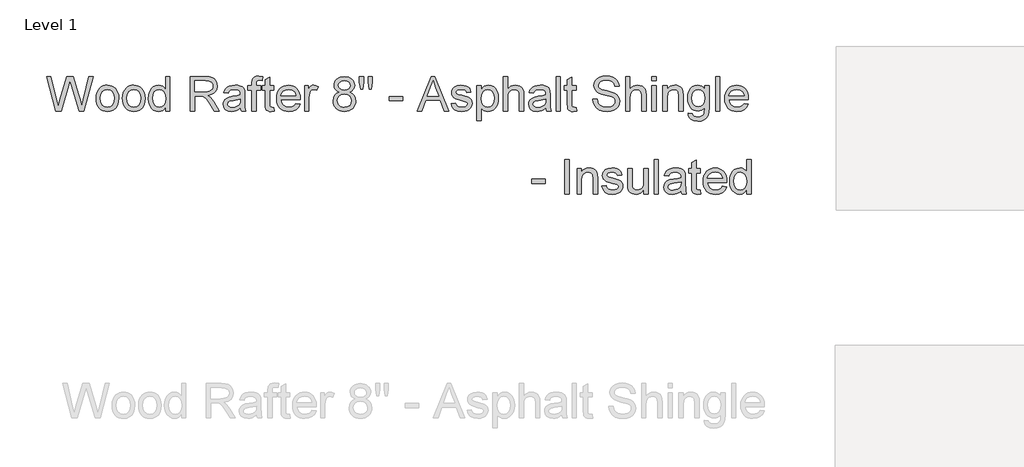
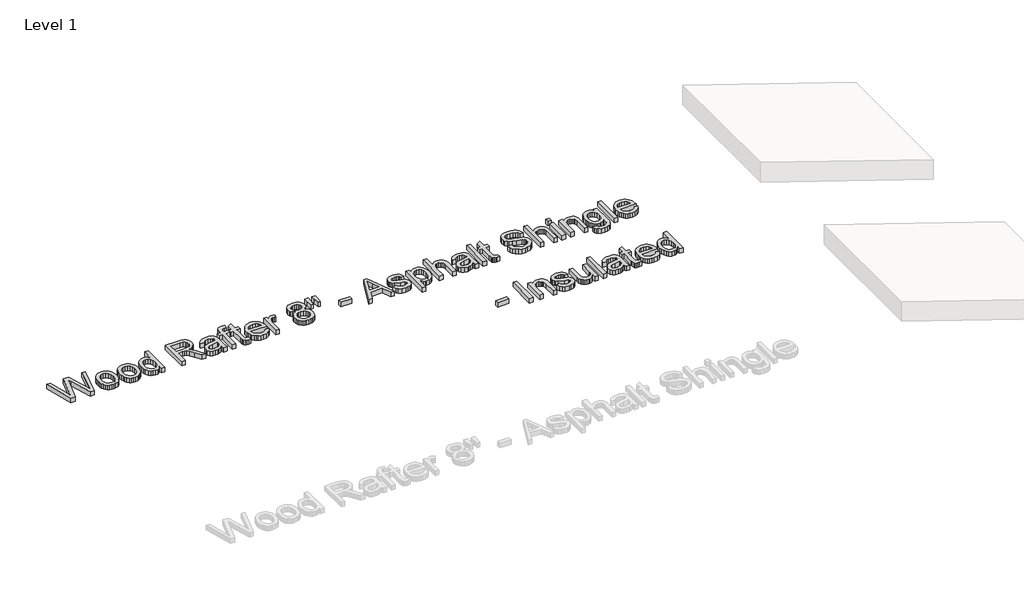
# One storey, part 9 of 42: 1 proxy.
"""IFC4 building model written with IfcOpenShell, lengths in millimetres."""

from ifc_helpers import new_model, si_unit, origin, origin_with_axes, place, context, project, spatial, polyline, outline, extrude, element, save

model = new_model("IFC4")

# Units and contexts
model_context = context("Model", 3, world=origin())
ifc_project = project(units=[si_unit("LENGTHUNIT", "METRE", prefix="MILLI")], contexts=[model_context])

# Site, building, storey
site = spatial("IfcSite", under=ifc_project)
building = spatial("IfcBuilding", under=site)
storey = spatial("IfcBuildingStorey", under=building, Name="Level 1", Elevation=0.0)

# Proxy
placement = place(None, origin())
element("IfcBuildingElementProxy", 1, Name="8\" Arial", ObjectType="8\" Arial", at=placement, inside=storey, context=model_context, shape_type="SweptSolid", body=[
    extrude(outline(polyline([(-8268.0994706, -5719.6737469), (-8351.1564638, -5415.1066528), (-8311.8958618, -5415.1066528), (-8263.7123957, -5615.2762371), (-8248.8409556, -5677.0670709), (-8232.9285147, -5622.4145284), (-8172.5504677, -5415.1066528), (-8115.964638, -5415.1066528), (-8072.0938895, -5565.3825554), (-8053.3001071, -5621.150456), (-8039.4510784, -5677.0670709), (-8025.0257815, -5617.0608099), (-7976.3961722, -5415.1066528), (-7937.1355703, -5415.1066528), (-8020.2669207, -5719.6737469), (-8060.9403094, -5719.6737469), (-8133.9590805, -5484.7049927), (-8144.146017, -5451.9134672), (-8155.5970259, -5491.3971407), (-8222.1467206, -5719.6737469), (-8268.0994706, -5719.6737469)])), origin_with_axes(), (0.0, 0.0, 1.0), 50.8),
    extrude(outline(polyline([(-7913.341266, -5607.840517), (-7911.2825011, -5578.87374), (-7905.1062061, -5553.9129572), (-7894.8123811, -5532.9581686), (-7880.4010261, -5516.0093742), (-7865.8920774, -5505.1764595), (-7849.8773953, -5497.4386633), (-7832.3569798, -5492.7959856), (-7813.3308311, -5491.2484263), (-7792.3272456, -5493.1329167), (-7773.3359518, -5498.7863876), (-7756.3569497, -5508.2088391), (-7741.3902394, -5521.4002712), (-7729.1747456, -5537.9145408), (-7720.4493928, -5557.3055045), (-7715.2141811, -5579.5731625), (-7713.4691106, -5604.7175146), (-7716.5549344, -5643.1787767), (-7725.8124059, -5672.4569245), (-7740.9719802, -5694.383004), (-7761.7641124, -5710.7880614), (-7786.4599977, -5721.0214712), (-7813.3308311, -5724.4326077), (-7834.6411401, -5722.5550884), (-7853.8090322, -5716.9225305), (-7870.8345075, -5707.5349339), (-7885.717566, -5694.3922987), (-7897.8029348, -5677.7176964), (-7906.435341, -5657.7341987), (-7911.6147848, -5634.4418056), (-7913.341266, -5607.840517)]), holes=[polyline([(-7875.2703793, -5607.7661598), (-7870.8647151, -5642.2214277), (-7857.6477227, -5666.7685986), (-7837.7571715, -5681.4634404), (-7813.3308311, -5686.361721), (-7789.0160265, -5681.4355564), (-7769.1626539, -5666.6570628), (-7755.9456615, -5641.7845792), (-7751.5399973, -5606.5764446), (-7755.9735454, -5573.124999), (-7769.2741897, -5548.9124355), (-7789.1554462, -5534.2175937), (-7813.3308311, -5529.3193131), (-7837.7571715, -5534.1990044), (-7857.6477227, -5548.8380783), (-7870.8647151, -5573.3294813), (-7875.2703793, -5607.7661598)])]), origin_with_axes(), (0.0, 0.0, 1.0), 50.8),
    extrude(outline(polyline([(-7680.1570847, -5607.840517), (-7678.0983197, -5578.87374), (-7671.9220247, -5553.9129572), (-7661.6281997, -5532.9581686), (-7647.2168447, -5516.0093742), (-7632.707896, -5505.1764595), (-7616.6932139, -5497.4386633), (-7599.1727984, -5492.7959856), (-7580.1466497, -5491.2484263), (-7559.1430642, -5493.1329167), (-7540.1517704, -5498.7863876), (-7523.1727683, -5508.2088391), (-7508.206058, -5521.4002712), (-7495.9905642, -5537.9145408), (-7487.2652114, -5557.3055045), (-7482.0299997, -5579.5731625), (-7480.2849292, -5604.7175146), (-7483.370753, -5643.1787767), (-7492.6282245, -5672.4569245), (-7507.7877988, -5694.383004), (-7528.579931, -5710.7880614), (-7553.2758163, -5721.0214712), (-7580.1466497, -5724.4326077), (-7601.4569587, -5722.5550884), (-7620.6248508, -5716.9225305), (-7637.6503261, -5707.5349339), (-7652.5333846, -5694.3922987), (-7664.6187534, -5677.7176964), (-7673.2511596, -5657.7341987), (-7678.4306034, -5634.4418056), (-7680.1570847, -5607.840517)]), holes=[polyline([(-7642.0861979, -5607.7661598), (-7637.6805338, -5642.2214277), (-7624.4635413, -5666.7685986), (-7604.5729901, -5681.4634404), (-7580.1466497, -5686.361721), (-7555.8318451, -5681.4355564), (-7535.9784725, -5666.6570628), (-7522.7614801, -5641.7845792), (-7518.3558159, -5606.5764446), (-7522.789364, -5573.124999), (-7536.0900083, -5548.9124355), (-7555.9712648, -5534.2175937), (-7580.1466497, -5529.3193131), (-7604.5729901, -5534.1990044), (-7624.4635413, -5548.8380783), (-7637.6805338, -5573.3294813), (-7642.0861979, -5607.7661598)])]), origin_with_axes(), (0.0, 0.0, 1.0), 50.8),
    extrude(outline(polyline([(-7299.4482171, -5719.6737469), (-7299.4482171, -5683.759219), (-7310.8388107, -5701.5538266), (-7324.6367188, -5714.2642605), (-7340.8419412, -5721.8905209), (-7359.454478, -5724.4326077), (-7384.0667115, -5720.7519263), (-7406.5969433, -5709.709882), (-7425.6695653, -5692.0779308), (-7439.9089692, -5668.6275286), (-7448.7760654, -5640.3067298), (-7451.7317641, -5608.0635886), (-7449.0084316, -5576.2201174), (-7440.8384342, -5547.4624701), (-7427.2310665, -5523.4265049), (-7408.1956231, -5505.7480805), (-7385.1727748, -5494.8733399), (-7359.6031924, -5491.2484263), (-7340.9767137, -5493.8416337), (-7324.5065937, -5501.6212558), (-7310.5460293, -5513.5462919), (-7299.4482171, -5528.5757411), (-7299.4482171, -5415.1066528), (-7261.3773303, -5415.1066528), (-7261.3773303, -5719.6737469), (-7299.4482171, -5719.6737469)]), holes=[polyline([(-7413.6608773, -5607.9148742), (-7409.366749, -5642.3515528), (-7396.484364, -5666.8429558), (-7377.7649387, -5681.4820297), (-7355.9596896, -5686.361721), (-7334.1637351, -5681.7051013), (-7315.918337, -5667.7352422), (-7303.5657471, -5644.1918935), (-7299.4482171, -5610.8148051), (-7303.6401043, -5574.3240088), (-7316.2157658, -5549.0239713), (-7334.9258965, -5534.2454777), (-7357.5211908, -5529.3193131), (-7379.5495115, -5534.05029), (-7397.599722, -5548.2432207), (-7409.6455885, -5572.6230879), (-7413.6608773, -5607.9148742)])]), origin_with_axes(), (0.0, 0.0, 1.0), 50.8),
    extrude(outline(polyline([(-7080.5406182, -5719.6737469), (-7080.5406182, -5415.1066528), (-6949.300159, -5415.1066528), (-6914.0269619, -5417.1607705), (-6888.364433, -5423.3231235), (-6869.6078291, -5434.6997752), (-6855.0524071, -5452.396789), (-6845.7112837, -5474.3414578), (-6842.597576, -5498.4610748), (-6847.7561068, -5528.4642053), (-6863.2316992, -5553.3366889), (-6874.9545766, -5563.4725049), (-6889.4890857, -5571.5727924), (-6926.9929988, -5581.6667824), (-6905.3550534, -5597.9510093), (-6874.4968151, -5637.1372541), (-6823.710847, -5719.6737469), (-6867.9533814, -5719.6737469), (-6907.5857694, -5656.5444835), (-6936.2132916, -5614.7557367), (-6956.3269144, -5595.0138999), (-6974.4328928, -5587.7640729), (-6996.5169814, -5586.4256432), (-7042.4697314, -5586.4256432), (-7042.4697314, -5719.6737469), (-7080.5406182, -5719.6737469)]), holes=[polyline([(-7042.4697314, -5548.3547565), (-6957.2563794, -5548.3547565), (-6932.7835658, -5547.0070322), (-6913.7945956, -5542.9638594), (-6899.4994238, -5535.9556933), (-6889.108005, -5525.7129889), (-6882.7783483, -5513.3232203), (-6880.6684627, -5499.8738616), (-6884.6930462, -5481.3031508), (-6896.7667967, -5466.3387641), (-6917.5403396, -5456.4678457), (-6947.6643006, -5453.1775396), (-7042.4697314, -5453.1775396), (-7042.4697314, -5548.3547565)])]), origin_with_axes(), (0.0, 0.0, 1.0), 50.8),
    extrude(outline(polyline([(-6637.9665596, -5691.1205818), (-6656.1561899, -5706.7170047), (-6674.8849098, -5716.9225305), (-6694.5802733, -5722.5550884), (-6715.6698344, -5724.4326077), (-6747.4854216, -5719.9154078), (-6770.9544131, -5706.363808), (-6785.4261833, -5685.7854527), (-6790.2501067, -5660.1879863), (-6788.4283553, -5644.4056705), (-6782.963101, -5630.0733201), (-6774.5328534, -5617.8043819), (-6763.8161218, -5608.212303), (-6737.1590654, -5595.7202933), (-6704.2188255, -5589.9947889), (-6665.2928309, -5583.9718556), (-6638.1896312, -5576.9079216), (-6637.9665596, -5568.4312007), (-6640.587651, -5551.4405803), (-6648.4509249, -5540.3241788), (-6666.0364029, -5532.0705295), (-6690.5371005, -5529.3193131), (-6713.2160467, -5531.1503592), (-6729.0541305, -5536.6434974), (-6739.8545139, -5546.8025499), (-6747.4203591, -5562.631339), (-6785.4912458, -5557.8724782), (-6778.8827496, -5537.052462), (-6769.0211259, -5520.6938778), (-6754.9862042, -5508.1832788), (-6735.8578144, -5498.907218), (-6712.4631801, -5493.1631243), (-6685.6295253, -5491.2484263), (-6659.8926392, -5492.9400527), (-6639.4908823, -5498.0149316), (-6624.1082364, -5505.6458393), (-6613.4286834, -5515.005552), (-6606.34616, -5526.5773913), (-6601.7546029, -5540.8446792), (-6599.8956729, -5574.1567051), (-6599.8956729, -5621.522242), (-6597.9623857, -5687.662972), (-6590.3779512, -5719.6737469), (-6628.4488379, -5719.6737469), (-6634.5461284, -5706.4381652), (-6637.9665596, -5691.1205818)]), holes=[polyline([(-6637.9665596, -5614.9788083), (-6699.3856074, -5626.6528888), (-6732.1399543, -5632.8245365), (-6746.9742159, -5642.8627586), (-6752.1792199, -5657.5111271), (-6749.3443516, -5668.8320109), (-6740.8397468, -5678.1080717), (-6726.8512984, -5684.2983087), (-6707.5648995, -5686.361721), (-6687.1166693, -5684.0845317), (-6669.0478695, -5677.2529639), (-6654.399501, -5667.1868579), (-6644.2125645, -5655.2060539), (-6639.6953646, -5642.8627586), (-6638.1896312, -5625.7606024), (-6637.9665596, -5614.9788083)])]), origin_with_axes(), (0.0, 0.0, 1.0), 50.8),
    extrude(outline(polyline([(-6538.0304819, -5719.6737469), (-6538.0304819, -5534.0781739), (-6571.3425078, -5534.0781739), (-6571.3425078, -5496.0072872), (-6538.0304819, -5496.0072872), (-6538.0304819, -5473.4770554), (-6534.0151931, -5441.7265307), (-6526.3564014, -5429.0672173), (-6514.5336065, -5419.0475845), (-6497.9891293, -5412.5227401), (-6476.1652909, -5410.347792), (-6441.4404782, -5414.5117952), (-6447.0172682, -5450.2032516), (-6468.9526424, -5448.4186787), (-6483.4244126, -5449.9987693), (-6492.9328397, -5454.7390408), (-6498.2029063, -5463.79203), (-6499.9595951, -5478.3102734), (-6499.9595951, -5496.0072872), (-6457.1298475, -5496.0072872), (-6457.1298475, -5534.0781739), (-6499.9595951, -5534.0781739), (-6499.9595951, -5719.6737469), (-6538.0304819, -5719.6737469)])), origin_with_axes(), (0.0, 0.0, 1.0), 50.8),
    extrude(outline(polyline([(-6342.9171873, -5687.9232222), (-6338.1583264, -5720.7891049), (-6366.6371343, -5724.4326077), (-6384.9104164, -5722.8525172), (-6398.5363734, -5718.1122457), (-6408.1656309, -5710.8066507), (-6414.4488143, -5701.5305899), (-6417.9064242, -5685.5995597), (-6419.0589608, -5658.3290563), (-6419.0589608, -5534.0781739), (-6447.6121258, -5534.0781739), (-6447.6121258, -5496.0072872), (-6419.0589608, -5496.0072872), (-6419.0589608, -5441.6521735), (-6380.988074, -5419.2706561), (-6380.988074, -5496.0072872), (-6342.9171873, -5496.0072872), (-6342.9171873, -5534.0781739), (-6380.988074, -5534.0781739), (-6380.988074, -5657.2136983), (-6378.9804296, -5676.8439993), (-6372.4741745, -5683.7963976), (-6359.498843, -5686.361721), (-6342.9171873, -5687.9232222)])), origin_with_axes(), (0.0, 0.0, 1.0), 50.8),
    extrude(outline(polyline([(-6148.2500358, -5653.0496951), (-6110.9227211, -5657.8085559), (-6124.3720798, -5685.9341671), (-6145.8334268, -5706.9586656), (-6174.8234404, -5720.0641222), (-6210.8587988, -5724.4326077), (-6234.481152, -5722.5481174), (-6255.5288871, -5716.8946465), (-6274.0020042, -5707.472195), (-6289.9005032, -5694.2807629), (-6302.6852944, -5677.6874888), (-6311.8172881, -5658.0595115), (-6317.2964843, -5635.3968309), (-6319.122883, -5609.6994471), (-6317.277895, -5583.1306898), (-6311.7429309, -5559.7128189), (-6302.5179907, -5539.4458344), (-6289.6030744, -5522.3297362), (-6273.7464013, -5508.7316632), (-6255.6961908, -5499.0187538), (-6235.4524429, -5493.1910082), (-6213.0151576, -5491.2484263), (-6191.3005314, -5493.1863609), (-6171.6632594, -5499.0001645), (-6154.1033417, -5508.6898372), (-6138.6207783, -5522.255379), (-6125.9823779, -5539.3342986), (-6116.954949, -5559.5641045), (-6111.5384916, -5582.9447968), (-6109.7330059, -5609.4763755), (-6109.9560775, -5619.7376692), (-6281.0519963, -5619.7376692), (-6274.4620894, -5648.2350663), (-6259.1538007, -5669.1852076), (-6237.0604174, -5682.0675926), (-6210.1152268, -5686.361721), (-6189.8528896, -5684.3726659), (-6172.7879121, -5678.4055005), (-6158.9202941, -5668.0884389), (-6148.2500358, -5653.0496951)]), holes=[polyline([(-6281.0519963, -5581.6667824), (-6147.8038926, -5581.6667824), (-6152.9531288, -5561.5531596), (-6163.0471188, -5547.1650413), (-6185.2427432, -5533.7807451), (-6213.163872, -5529.3193131), (-6238.8264009, -5532.8791641), (-6260.0460871, -5543.558717), (-6274.7966968, -5560.2054353), (-6281.0519963, -5581.6667824)])]), origin_with_axes(), (0.0, 0.0, 1.0), 50.8),
    extrude(outline(polyline([(-6071.6621191, -5719.6737469), (-6071.6621191, -5496.0072872), (-6038.3500932, -5496.0072872), (-6038.3500932, -5529.0962415), (-6026.0439765, -5509.9120837), (-6014.7045034, -5498.6097892), (-6003.3278517, -5493.0887671), (-5990.9101991, -5491.2484263), (-5971.949113, -5494.1855358), (-5952.690598, -5502.9968641), (-5965.4056793, -5537.1268192), (-5978.7899754, -5531.2711896), (-5992.1742716, -5529.3193131), (-6003.5416286, -5531.1968324), (-6013.7006812, -5536.8293904), (-6021.9078572, -5545.7894331), (-6027.4195847, -5557.6494066), (-6032.0483204, -5578.915566), (-6033.5912323, -5602.1150126), (-6033.5912323, -5719.6737469), (-6071.6621191, -5719.6737469)])), origin_with_axes(), (0.0, 0.0, 1.0), 50.8),
    extrude(outline(polyline([(-5763.9720226, -5551.9239021), (-5784.3551902, -5541.88568), (-5798.6596567, -5528.2783123), (-5807.1084937, -5511.3806384), (-5809.9247726, -5491.4714979), (-5808.3911554, -5475.944785), (-5803.7903036, -5461.7100284), (-5796.1222173, -5448.7672281), (-5785.3868964, -5437.1163842), (-5772.1001941, -5427.4871267), (-5756.7779634, -5420.6090857), (-5720.026917, -5415.1066528), (-5683.0527989, -5420.7392108), (-5667.5632646, -5427.7799082), (-5654.07208, -5437.6368846), (-5643.1415715, -5449.5154475), (-5635.3340654, -5462.6209041), (-5630.6495618, -5476.9532545), (-5629.0880605, -5492.5124988), (-5631.8671609, -5511.7803084), (-5640.204462, -5528.3898481), (-5654.1929104, -5541.913564), (-5673.9254526, -5551.9239021), (-5650.4936397, -5563.9976526), (-5633.4379568, -5581.7783182), (-5623.0372433, -5604.4107912), (-5619.5703388, -5631.0399637), (-5621.2898491, -5650.0289338), (-5626.4483799, -5667.4378134), (-5635.0459312, -5683.2666025), (-5647.0825031, -5697.5153011), (-5661.9260593, -5709.2916227), (-5678.9445636, -5717.7032811), (-5698.138016, -5722.7502761), (-5719.5064166, -5724.4326077), (-5740.8748171, -5722.7433051), (-5760.0682696, -5717.6753971), (-5777.0867739, -5709.2288839), (-5791.9303301, -5697.4037653), (-5803.9669019, -5683.0551492), (-5812.5644533, -5667.0381435), (-5817.7229841, -5649.352748), (-5819.4424943, -5629.9989629), (-5815.8361701, -5602.3380842), (-5805.0171974, -5579.5847808), (-5787.5432552, -5562.5198032), (-5763.9720226, -5551.9239021)]), holes=[polyline([(-5771.8538859, -5492.586856), (-5768.4799279, -5509.2056903), (-5758.358054, -5522.4784506), (-5741.7856928, -5531.1782431), (-5719.0602734, -5534.0781739), (-5696.864649, -5531.1968324), (-5680.5432434, -5522.5528078), (-5670.5050213, -5509.7261907), (-5667.1589473, -5494.2970716), (-5670.6165571, -5478.2823895), (-5680.9893866, -5465.0375131), (-5697.5338638, -5456.142533), (-5719.5064166, -5453.1775396), (-5741.6183891, -5456.0774704), (-5758.1349824, -5464.7772629), (-5768.42416, -5477.5295228), (-5771.8538859, -5492.586856)]), polyline([(-5781.3716076, -5628.6605332), (-5779.7822224, -5643.2252499), (-5775.0140669, -5657.3252341), (-5766.2120333, -5669.6220562), (-5752.5210137, -5678.7772865), (-5736.1252509, -5684.4656124), (-5719.2089878, -5686.361721), (-5693.2955033, -5682.3743161), (-5673.8510954, -5670.4121014), (-5661.693693, -5652.2968284), (-5657.6412256, -5629.8502485), (-5661.8238181, -5607.0225878), (-5674.3715958, -5588.5076449), (-5694.2621469, -5576.2387067), (-5720.4730602, -5572.1490607), (-5746.0240533, -5576.1829388), (-5765.2732736, -5588.2845733), (-5777.3470241, -5606.4463195), (-5781.3716076, -5628.6605332)])]), origin_with_axes(), (0.0, 0.0, 1.0), 50.8),
    extrude(outline(polyline([(-5576.9636628, -5524.5604523), (-5586.2583129, -5465.7439065), (-5586.2583129, -5415.1066528), (-5548.1874262, -5415.1066528), (-5548.1874262, -5465.7439065), (-5556.5154327, -5524.5604523), (-5576.9636628, -5524.5604523)])), origin_with_axes(), (0.0, 0.0, 1.0), 50.8),
    extrude(outline(polyline([(-5501.0449609, -5524.5604523), (-5510.1165394, -5465.7439065), (-5510.1165394, -5415.1066528), (-5472.0456527, -5415.1066528), (-5472.0456527, -5465.7439065), (-5480.9685167, -5524.5604523), (-5501.0449609, -5524.5604523)])), origin_with_axes(), (0.0, 0.0, 1.0), 50.8),
    extrude(outline(polyline([(-5324.5209665, -5629.2553908), (-5324.5209665, -5591.1845041), (-5205.5494453, -5591.1845041), (-5205.5494453, -5629.2553908), (-5324.5209665, -5629.2553908)])), origin_with_axes(), (0.0, 0.0, 1.0), 50.8),
    extrude(outline(polyline([(-5074.4577005, -5719.6737469), (-4952.8836774, -5415.1066528), (-4920.4639379, -5415.1066528), (-4798.8899147, -5719.6737469), (-4839.1171603, -5719.6737469), (-4873.9906874, -5624.49653), (-4999.431285, -5624.49653), (-5034.2304549, -5719.6737469), (-5074.4577005, -5719.6737469)]), holes=[polyline([(-4985.4521313, -5586.4256432), (-4887.895484, -5586.4256432), (-4915.333291, -5511.5479421), (-4936.6738076, -5453.1775396), (-4955.6348938, -5505.0045085), (-4985.4521313, -5586.4256432)])]), origin_with_axes(), (0.0, 0.0, 1.0), 50.8),
    extrude(outline(polyline([(-4777.2519693, -5653.0496951), (-4739.1810826, -5648.2908342), (-4733.1767386, -5664.5750612), (-4721.558426, -5676.5465705), (-4704.2517875, -5683.9079334), (-4681.182466, -5686.361721), (-4658.391984, -5684.1124157), (-4642.3680072, -5677.3644997), (-4632.8874642, -5667.5865278), (-4629.7272831, -5656.2470547), (-4632.9060535, -5646.54344), (-4642.4423644, -5639.1448985), (-4681.6286092, -5628.2887472), (-4738.958011, -5609.6622685), (-4753.4669597, -5600.3025558), (-4763.979209, -5587.9127873), (-4770.3646336, -5573.283008), (-4772.4931085, -5557.2032634), (-4770.7828929, -5542.4526537), (-4765.652246, -5528.8359913), (-4757.5659004, -5516.8923659), (-4746.9885886, -5507.1608673), (-4722.7853198, -5495.8957514), (-4690.0309729, -5491.2484263), (-4665.2514358, -5493.116651), (-4643.7064369, -5498.721325), (-4626.3812091, -5507.514064), (-4614.2609854, -5518.9464836), (-4606.2304077, -5533.864397), (-4601.1741181, -5553.1136173), (-4639.2450048, -5557.8724782), (-4644.0503389, -5545.8916742), (-4653.5587659, -5536.866569), (-4667.8632324, -5531.2061271), (-4687.0566849, -5529.3193131), (-4708.9177019, -5531.1224752), (-4723.4917132, -5536.5319616), (-4731.6895946, -5544.3394676), (-4734.4222217, -5553.3366889), (-4729.8864325, -5564.4159118), (-4715.6842071, -5572.8182755), (-4682.8926816, -5580.9232104), (-4627.0132453, -5598.8432958), (-4612.253341, -5607.4129631), (-4601.0625823, -5619.1428115), (-4594.0079428, -5634.0700196), (-4591.6563964, -5652.2317659), (-4594.4169074, -5671.006959), (-4602.6984407, -5688.6667942), (-4616.1849779, -5703.8263685), (-4634.5605012, -5715.1007791), (-4656.7561256, -5722.0996506), (-4681.7029664, -5724.4326077), (-4720.0898713, -5719.9339971), (-4748.1039466, -5706.4381652), (-4766.8047826, -5684.0938264), (-4777.2519693, -5653.0496951)])), origin_with_axes(), (0.0, 0.0, 1.0), 50.8),
    extrude(outline(polyline([(-4548.8266488, -5805.3332421), (-4548.8266488, -5496.0072872), (-4510.755762, -5496.0072872), (-4510.755762, -5533.3346019), (-4498.3381095, -5514.9219001), (-4484.433313, -5501.7699702), (-4468.2234432, -5493.8788123), (-4448.890571, -5491.2484263), (-4423.1443903, -5494.9291078), (-4400.6327478, -5505.9711521), (-4382.3036978, -5523.7053445), (-4369.1052947, -5547.4624701), (-4361.1304849, -5575.513724), (-4358.472215, -5606.1303014), (-4361.4743869, -5638.6894607), (-4370.4809029, -5667.8095994), (-4385.2036286, -5692.0128682), (-4405.35443, -5709.8214178), (-4428.8234215, -5720.7798103), (-4453.5007175, -5724.4326077), (-4471.0025436, -5721.9881148), (-4486.6268504, -5714.6546358), (-4500.0018519, -5703.5847076), (-4510.755762, -5689.9308666), (-4510.755762, -5805.3332421), (-4548.8266488, -5805.3332421)]), holes=[polyline([(-4510.755762, -5609.6250899), (-4506.638232, -5643.755045), (-4494.285642, -5667.6237064), (-4476.0588332, -5681.6772173), (-4454.3186467, -5686.361721), (-4432.2252634, -5681.5099136), (-4413.5337221, -5666.9544916), (-4400.7907568, -5642.2121331), (-4396.5431017, -5606.7995162), (-4400.6885157, -5572.8554541), (-4413.1247575, -5548.6521853), (-4431.3236824, -5534.1525311), (-4452.7571455, -5529.3193131), (-4474.2742604, -5534.4592546), (-4493.170284, -5549.8790791), (-4506.3593925, -5575.0954648), (-4510.755762, -5609.6250899)])]), origin_with_axes(), (0.0, 0.0, 1.0), 50.8),
    extrude(outline(polyline([(-4315.6424674, -5719.6737469), (-4315.6424674, -5415.1066528), (-4277.5715806, -5415.1066528), (-4277.5715806, -5527.0885971), (-4263.5877796, -5511.4085224), (-4247.8844682, -5500.208469), (-4230.4616466, -5493.488437), (-4211.3193148, -5491.2484263), (-4188.3243505, -5493.6929193), (-4168.5639244, -5501.0263982), (-4153.0046801, -5512.6725948), (-4142.6132613, -5528.0552407), (-4136.7576318, -5549.191275), (-4134.8057553, -5578.0976368), (-4134.8057553, -5719.6737469), (-4172.876642, -5719.6737469), (-4172.876642, -5582.0385684), (-4175.906698, -5558.2070856), (-4184.9968657, -5541.88568), (-4199.6452343, -5532.4609048), (-4219.3498925, -5529.3193131), (-4235.4389318, -5531.4384933), (-4250.5427382, -5537.796034), (-4263.0533372, -5547.7784882), (-4271.3627543, -5560.772409), (-4276.019374, -5578.0418689), (-4277.5715806, -5600.8509402), (-4277.5715806, -5719.6737469), (-4315.6424674, -5719.6737469)])), origin_with_axes(), (0.0, 0.0, 1.0), 50.8),
    extrude(outline(polyline([(-3939.6924606, -5691.1205818), (-3957.8820908, -5706.7170047), (-3976.6108108, -5716.9225305), (-3996.3061743, -5722.5550884), (-4017.3957354, -5724.4326077), (-4049.2113226, -5719.9154078), (-4072.6803141, -5706.363808), (-4087.1520843, -5685.7854527), (-4091.9760077, -5660.1879863), (-4090.1542562, -5644.4056705), (-4084.689002, -5630.0733201), (-4076.2587544, -5617.8043819), (-4065.5420228, -5608.212303), (-4038.8849664, -5595.7202933), (-4005.9447264, -5589.9947889), (-3967.0187319, -5583.9718556), (-3939.9155322, -5576.9079216), (-3939.6924606, -5568.4312007), (-3942.313552, -5551.4405803), (-3950.1768259, -5540.3241788), (-3967.7623039, -5532.0705295), (-3992.2630015, -5529.3193131), (-4014.9419477, -5531.1503592), (-4030.7800315, -5536.6434974), (-4041.5804149, -5546.8025499), (-4049.1462601, -5562.631339), (-4087.2171468, -5557.8724782), (-4080.6086506, -5537.052462), (-4070.7470269, -5520.6938778), (-4056.7121052, -5508.1832788), (-4037.5837153, -5498.907218), (-4014.1890811, -5493.1631243), (-3987.3554263, -5491.2484263), (-3961.6185402, -5492.9400527), (-3941.2167832, -5498.0149316), (-3925.8341373, -5505.6458393), (-3915.1545844, -5515.005552), (-3908.072061, -5526.5773913), (-3903.4805039, -5540.8446792), (-3901.6215739, -5574.1567051), (-3901.6215739, -5621.522242), (-3899.6882866, -5687.662972), (-3892.1038522, -5719.6737469), (-3930.1747389, -5719.6737469), (-3936.2720294, -5706.4381652), (-3939.6924606, -5691.1205818)]), holes=[polyline([(-3939.6924606, -5614.9788083), (-4001.1115084, -5626.6528888), (-4033.8658553, -5632.8245365), (-4048.7001169, -5642.8627586), (-4053.9051209, -5657.5111271), (-4051.0702526, -5668.8320109), (-4042.5656478, -5678.1080717), (-4028.5771994, -5684.2983087), (-4009.2908005, -5686.361721), (-3988.8425703, -5684.0845317), (-3970.7737705, -5677.2529639), (-3956.125402, -5667.1868579), (-3945.9384655, -5655.2060539), (-3941.4212655, -5642.8627586), (-3939.9155322, -5625.7606024), (-3939.6924606, -5614.9788083)])]), origin_with_axes(), (0.0, 0.0, 1.0), 50.8),
    extrude(outline(polyline([(-3849.2741046, -5719.6737469), (-3849.2741046, -5415.1066528), (-3811.2032178, -5415.1066528), (-3811.2032178, -5719.6737469), (-3849.2741046, -5719.6737469)])), origin_with_axes(), (0.0, 0.0, 1.0), 50.8),
    extrude(outline(polyline([(-3673.1962533, -5687.9232222), (-3668.4373925, -5720.7891049), (-3696.9162003, -5724.4326077), (-3715.1894824, -5722.8525172), (-3728.8154394, -5718.1122457), (-3738.4446969, -5710.8066507), (-3744.7278804, -5701.5305899), (-3748.1854902, -5685.5995597), (-3749.3380268, -5658.3290563), (-3749.3380268, -5534.0781739), (-3777.8911919, -5534.0781739), (-3777.8911919, -5496.0072872), (-3749.3380268, -5496.0072872), (-3749.3380268, -5441.6521735), (-3711.2671401, -5419.2706561), (-3711.2671401, -5496.0072872), (-3673.1962533, -5496.0072872), (-3673.1962533, -5534.0781739), (-3711.2671401, -5534.0781739), (-3711.2671401, -5657.2136983), (-3709.2594957, -5676.8439993), (-3702.7532406, -5683.7963976), (-3689.7779091, -5686.361721), (-3673.1962533, -5687.9232222)])), origin_with_axes(), (0.0, 0.0, 1.0), 50.8),
    extrude(outline(polyline([(-3525.6715671, -5614.9788083), (-3487.6006804, -5614.9788083), (-3483.2321948, -5636.105548), (-3475.3317423, -5653.0868737), (-3463.0070362, -5666.5641163), (-3445.3657904, -5677.1786067), (-3423.8022022, -5684.0659424), (-3399.7104691, -5686.361721), (-3378.5000776, -5684.6236214), (-3359.9293668, -5679.4093227), (-3344.8813283, -5671.1556734), (-3334.2389539, -5660.2995221), (-3327.9092972, -5647.8353964), (-3325.7994116, -5634.7578237), (-3327.3795022, -5622.0148584), (-3332.1197737, -5611.0006981), (-3341.7490312, -5601.6038068), (-3357.9960795, -5593.7126489), (-3413.4293727, -5579.1758162), (-3449.8179278, -5569.5558533), (-3473.1010262, -5560.400623), (-3492.0528178, -5547.5925952), (-3505.4835871, -5532.0705295), (-3513.4862809, -5514.1690335), (-3516.1538454, -5494.2227144), (-3512.8542447, -5471.9248488), (-3502.9554423, -5451.1327166), (-3486.7176886, -5433.51006), (-3464.4012337, -5420.7206215), (-3437.6140522, -5412.9409994), (-3407.9641184, -5410.347792), (-3375.8418077, -5413.0618298), (-3347.7347859, -5421.2039433), (-3324.646875, -5434.6068287), (-3307.5818975, -5453.1031824), (-3296.7815141, -5475.5404677), (-3292.4873857, -5500.766148), (-3330.5582725, -5500.766148), (-3337.5478494, -5478.0500232), (-3352.1218607, -5461.6542605), (-3374.8937534, -5451.7275742), (-3406.4769744, -5448.4186787), (-3438.8037674, -5451.6903956), (-3460.9808025, -5461.5055461), (-3473.8074196, -5475.9494323), (-3478.0829587, -5493.1073564), (-3475.0529028, -5507.7371356), (-3465.962735, -5519.5041626), (-3444.473504, -5530.0257065), (-3403.8001152, -5540.770322), (-3361.8254754, -5550.9758478), (-3336.4324913, -5559.8801226), (-3314.7294834, -5573.6919726), (-3299.5884984, -5590.7383609), (-3290.6935183, -5610.8333944), (-3287.7285249, -5633.7911801), (-3291.1396615, -5657.2601716), (-3301.3730712, -5679.3349655), (-3318.0104949, -5698.3332303), (-3340.6336732, -5712.5726342), (-3367.839114, -5721.4676144), (-3398.2233251, -5724.4326077), (-3435.5227559, -5721.2352481), (-3466.2229852, -5711.6431692), (-3490.6772095, -5695.6191925), (-3509.2386258, -5673.1261393), (-3521.1543672, -5645.7255108), (-3525.6715671, -5614.9788083)])), origin_with_axes(), (0.0, 0.0, 1.0), 50.8),
    extrude(outline(polyline([(-3235.3810556, -5719.6737469), (-3235.3810556, -5415.1066528), (-3197.3101688, -5415.1066528), (-3197.3101688, -5527.0885971), (-3183.3263678, -5511.4085224), (-3167.6230565, -5500.208469), (-3150.2002349, -5493.488437), (-3131.057903, -5491.2484263), (-3108.0629387, -5493.6929193), (-3088.3025126, -5501.0263982), (-3072.7432684, -5512.6725948), (-3062.3518496, -5528.0552407), (-3056.49622, -5549.191275), (-3054.5443435, -5578.0976368), (-3054.5443435, -5719.6737469), (-3092.6152302, -5719.6737469), (-3092.6152302, -5582.0385684), (-3095.6452862, -5558.2070856), (-3104.735454, -5541.88568), (-3119.3838225, -5532.4609048), (-3139.0884807, -5529.3193131), (-3155.17752, -5531.4384933), (-3170.2813264, -5537.796034), (-3182.7919254, -5547.7784882), (-3191.1013426, -5560.772409), (-3195.7579623, -5578.0418689), (-3197.3101688, -5600.8509402), (-3197.3101688, -5719.6737469), (-3235.3810556, -5719.6737469)])), origin_with_axes(), (0.0, 0.0, 1.0), 50.8),
    extrude(outline(polyline([(-3002.1968742, -5453.1775396), (-3002.1968742, -5415.1066528), (-2964.1259874, -5415.1066528), (-2964.1259874, -5453.1775396), (-3002.1968742, -5453.1775396)])), origin_with_axes(), (0.0, 0.0, 1.0), 50.8),
    extrude(outline(polyline([(-3002.1968742, -5719.6737469), (-3002.1968742, -5496.0072872), (-2964.1259874, -5496.0072872), (-2964.1259874, -5719.6737469), (-3002.1968742, -5719.6737469)])), origin_with_axes(), (0.0, 0.0, 1.0), 50.8),
    extrude(outline(polyline([(-2907.0196573, -5719.6737469), (-2907.0196573, -5496.0072872), (-2868.9487705, -5496.0072872), (-2868.9487705, -5527.2373115), (-2855.7224835, -5511.4921742), (-2839.8379265, -5500.2456476), (-2821.2950995, -5493.4977317), (-2800.0940027, -5491.2484263), (-2781.3281042, -5493.0608831), (-2764.1422962, -5498.4982534), (-2749.8099457, -5506.8820278), (-2739.6044199, -5517.5336968), (-2728.1905896, -5545.5291829), (-2726.1829452, -5582.3359972), (-2726.1829452, -5719.6737469), (-2764.253832, -5719.6737469), (-2764.253832, -5587.4666441), (-2768.6409068, -5553.7828321), (-2774.7103133, -5543.7539047), (-2784.1443831, -5535.9742826), (-2796.2367229, -5530.9830555), (-2810.2809392, -5529.3193131), (-2832.5788047, -5533.0557624), (-2851.5863642, -5544.2651104), (-2859.182417, -5553.4156935), (-2864.608169, -5565.9216451), (-2868.9487705, -5600.9996546), (-2868.9487705, -5719.6737469), (-2907.0196573, -5719.6737469)])), origin_with_axes(), (0.0, 0.0, 1.0), 50.8),
    extrude(outline(polyline([(-2683.3531976, -5738.7091903), (-2645.2823108, -5743.4680511), (-2641.081129, -5755.3652032), (-2632.9390155, -5763.5444953), (-2616.9336281, -5769.902036), (-2595.9834868, -5772.0212162), (-2573.639148, -5769.6231965), (-2557.0203136, -5762.4291373), (-2545.4949475, -5750.9037712), (-2538.4310134, -5735.5118306), (-2535.8285114, -5691.1205818), (-2548.4971195, -5703.6125915), (-2562.6342823, -5712.5354556), (-2578.2399998, -5717.8891741), (-2595.314272, -5719.6737469), (-2616.1877324, -5717.5963926), (-2634.5655793, -5711.3643297), (-2650.4478126, -5700.9775582), (-2663.8344324, -5686.4360782), (-2674.4558938, -5668.99002), (-2682.0426519, -5649.889514), (-2686.5947068, -5629.1345604), (-2688.1120584, -5606.725159), (-2685.388726, -5575.9877512), (-2677.2187285, -5547.7227203), (-2663.8902003, -5523.770407), (-2645.6912754, -5505.9711521), (-2623.2446955, -5494.9291078), (-2597.173202, -5491.2484263), (-2579.3692997, -5493.330428), (-2563.2105506, -5499.5764328), (-2548.6969545, -5509.9864409), (-2535.8285114, -5524.5604523), (-2535.8285114, -5496.0072872), (-2497.7576246, -5496.0072872), (-2497.7576246, -5689.1129374), (-2500.3601267, -5733.6993739), (-2508.1676327, -5763.0611735), (-2521.6169914, -5782.5334654), (-2541.1450513, -5797.4513788), (-2566.3242583, -5806.9319219), (-2596.7270588, -5810.0921029), (-2632.1489703, -5805.6399656), (-2660.0422152, -5792.2835534), (-2670.5474934, -5782.2569496), (-2677.9344166, -5769.9856878), (-2682.2029846, -5755.469768), (-2683.3531976, -5738.7091903)]), holes=[polyline([(-2650.0411717, -5604.122657), (-2645.9794096, -5639.0426574), (-2633.7941233, -5663.0507386), (-2615.474368, -5676.9648297), (-2593.0091987, -5681.6028601), (-2570.7113332, -5676.9927137), (-2552.2986314, -5663.1622744), (-2539.9460414, -5639.4609166), (-2535.8285114, -5605.238015), (-2540.0668718, -5572.2327126), (-2552.7819532, -5548.4662923), (-2571.4641998, -5534.1060579), (-2593.6040563, -5529.3193131), (-2615.3442429, -5534.0317007), (-2633.5710517, -5548.1688635), (-2645.9236417, -5571.5820871), (-2650.0411717, -5604.122657)])]), origin_with_axes(), (0.0, 0.0, 1.0), 50.8),
    extrude(outline(polyline([(-2440.6512945, -5719.6737469), (-2440.6512945, -5415.1066528), (-2402.5804077, -5415.1066528), (-2402.5804077, -5719.6737469), (-2440.6512945, -5719.6737469)])), origin_with_axes(), (0.0, 0.0, 1.0), 50.8),
    extrude(outline(polyline([(-2188.8778129, -5653.0496951), (-2151.5504982, -5657.8085559), (-2164.9998569, -5685.9341671), (-2186.4612039, -5706.9586656), (-2215.4512175, -5720.0641222), (-2251.4865759, -5724.4326077), (-2275.1089291, -5722.5481174), (-2296.1566642, -5716.8946465), (-2314.6297813, -5707.472195), (-2330.5282803, -5694.2807629), (-2343.3130715, -5677.6874888), (-2352.4450652, -5658.0595115), (-2357.9242614, -5635.3968309), (-2359.7506601, -5609.6994471), (-2357.9056721, -5583.1306898), (-2352.370708, -5559.7128189), (-2343.1457678, -5539.4458344), (-2330.2308515, -5522.3297362), (-2314.3741784, -5508.7316632), (-2296.3239679, -5499.0187538), (-2276.0802201, -5493.1910082), (-2253.6429347, -5491.2484263), (-2231.9283085, -5493.1863609), (-2212.2910365, -5499.0001645), (-2194.7311188, -5508.6898372), (-2179.2485554, -5522.255379), (-2166.610155, -5539.3342986), (-2157.5827261, -5559.5641045), (-2152.1662688, -5582.9447968), (-2150.360783, -5609.4763755), (-2150.5838546, -5619.7376692), (-2321.6797734, -5619.7376692), (-2315.0898665, -5648.2350663), (-2299.7815778, -5669.1852076), (-2277.6881945, -5682.0675926), (-2250.7430039, -5686.361721), (-2230.4806667, -5684.3726659), (-2213.4156892, -5678.4055005), (-2199.5480712, -5668.0884389), (-2188.8778129, -5653.0496951)]), holes=[polyline([(-2321.6797734, -5581.6667824), (-2188.4316697, -5581.6667824), (-2193.5809059, -5561.5531596), (-2203.6748959, -5547.1650413), (-2225.8705203, -5533.7807451), (-2253.7916491, -5529.3193131), (-2279.454178, -5532.8791641), (-2300.6738642, -5543.558717), (-2315.4244739, -5560.2054353), (-2321.6797734, -5581.6667824)])]), origin_with_axes(), (0.0, 0.0, 1.0), 50.8),
    extrude(outline(polyline([(-4063.4228426, -6361.3607195), (-4063.4228426, -6323.2898328), (-3944.4513215, -6323.2898328), (-3944.4513215, -6361.3607195), (-4063.4228426, -6361.3607195)])), origin_with_axes(), (0.0, 0.0, 1.0), 50.8),
    extrude(outline(polyline([(-3773.1323311, -6451.7790756), (-3773.1323311, -6147.2119815), (-3735.0614443, -6147.2119815), (-3735.0614443, -6451.7790756), (-3773.1323311, -6451.7790756)])), origin_with_axes(), (0.0, 0.0, 1.0), 50.8),
    extrude(outline(polyline([(-3663.6785316, -6451.7790756), (-3663.6785316, -6228.1126159), (-3625.6076449, -6228.1126159), (-3625.6076449, -6259.3426402), (-3612.3813578, -6243.5975029), (-3596.4968008, -6232.3509763), (-3577.9539739, -6225.6030603), (-3556.752877, -6223.353755), (-3537.9869785, -6225.1662118), (-3520.8011705, -6230.6035821), (-3506.46882, -6238.9873565), (-3496.2632942, -6249.6390255), (-3484.8494639, -6277.6345115), (-3482.8418195, -6314.4413259), (-3482.8418195, -6451.7790756), (-3520.9127063, -6451.7790756), (-3520.9127063, -6319.5719727), (-3525.2997811, -6285.8881608), (-3531.3691876, -6275.8592334), (-3540.8032575, -6268.0796112), (-3552.8955972, -6263.0883841), (-3566.9398135, -6261.4246418), (-3589.2376791, -6265.1610911), (-3608.2452385, -6276.3704391), (-3615.8412913, -6285.5210221), (-3621.2670433, -6298.0269738), (-3625.6076449, -6333.1049833), (-3625.6076449, -6451.7790756), (-3663.6785316, -6451.7790756)])), origin_with_axes(), (0.0, 0.0, 1.0), 50.8),
    extrude(outline(polyline([(-3444.7709328, -6385.1550237), (-3406.700046, -6380.3961629), (-3400.695702, -6396.6803899), (-3389.0773894, -6408.6518992), (-3371.770751, -6416.013262), (-3348.7014295, -6418.4670497), (-3325.9109474, -6416.2177443), (-3309.8869707, -6409.4698284), (-3300.4064276, -6399.6918565), (-3297.2462466, -6388.3523834), (-3300.4250169, -6378.6487687), (-3309.9613279, -6371.2502272), (-3349.1475727, -6360.3940759), (-3406.4769744, -6341.7675971), (-3420.9859232, -6332.4078845), (-3431.4981724, -6320.0181159), (-3437.8835971, -6305.3883367), (-3440.0120719, -6289.308592), (-3438.3018563, -6274.5579824), (-3433.1712095, -6260.94132), (-3425.0848639, -6248.9976946), (-3414.5075521, -6239.266196), (-3390.3042833, -6228.0010801), (-3357.5499363, -6223.353755), (-3332.7703992, -6225.2219797), (-3311.2254003, -6230.8266537), (-3293.9001725, -6239.6193927), (-3281.7799488, -6251.0518123), (-3273.7493712, -6265.9697257), (-3268.6930815, -6285.218946), (-3306.7639683, -6289.9778069), (-3311.5693024, -6277.9970029), (-3321.0777294, -6268.9718977), (-3335.3821959, -6263.3114557), (-3354.5756483, -6261.4246418), (-3376.4366653, -6263.2278039), (-3391.0106767, -6268.6372903), (-3399.208558, -6276.4447963), (-3401.9411852, -6285.4420176), (-3397.4053959, -6296.5212405), (-3383.2031706, -6304.9236042), (-3350.4116451, -6313.0285391), (-3294.5322088, -6330.9486244), (-3279.7723044, -6339.5182918), (-3268.5815457, -6351.2481402), (-3261.5269063, -6366.1753483), (-3259.1753598, -6384.3370945), (-3261.9358709, -6403.1122877), (-3270.2174041, -6420.7721229), (-3283.7039414, -6435.9316972), (-3302.0794646, -6447.2061077), (-3324.275089, -6454.2049792), (-3349.2219299, -6456.5379364), (-3387.6088347, -6452.0393258), (-3415.6229101, -6438.5434939), (-3434.3237461, -6416.199155), (-3444.7709328, -6385.1550237)])), origin_with_axes(), (0.0, 0.0, 1.0), 50.8),
    extrude(outline(polyline([(-3073.5797869, -6451.7790756), (-3073.5797869, -6413.3364028), (-3087.3544583, -6432.2370738), (-3103.3970244, -6445.737553), (-3121.707485, -6453.8378406), (-3142.2858403, -6456.5379364), (-3160.8286672, -6454.6418278), (-3178.0888325, -6448.9535019), (-3192.5698973, -6440.4024239), (-3202.7754231, -6429.9180586), (-3209.6441695, -6417.1843879), (-3214.1148962, -6401.8853939), (-3216.3456122, -6366.4913664), (-3216.3456122, -6228.1126159), (-3178.2747255, -6228.1126159), (-3178.2747255, -6348.571281), (-3175.9696522, -6387.3857398), (-3170.4207461, -6400.3331873), (-3160.9123191, -6410.1762218), (-3148.0764073, -6416.3943427), (-3132.545047, -6418.4670497), (-3116.1214003, -6416.3478694), (-3100.7573437, -6409.9903288), (-3088.0887357, -6399.9799906), (-3079.7514345, -6386.902418), (-3075.1226988, -6368.9916272), (-3073.5797869, -6344.481635), (-3073.5797869, -6228.1126159), (-3035.5089001, -6228.1126159), (-3035.5089001, -6451.7790756), (-3073.5797869, -6451.7790756)])), origin_with_axes(), (0.0, 0.0, 1.0), 50.8),
    extrude(outline(polyline([(-2983.1614308, -6451.7790756), (-2983.1614308, -6147.2119815), (-2945.0905441, -6147.2119815), (-2945.0905441, -6451.7790756), (-2983.1614308, -6451.7790756)])), origin_with_axes(), (0.0, 0.0, 1.0), 50.8),
    extrude(outline(polyline([(-2745.2183886, -6423.2259105), (-2763.4080188, -6438.8223334), (-2782.1367387, -6449.0278591), (-2801.8321023, -6454.6604171), (-2822.9216633, -6456.5379364), (-2854.7372506, -6452.0207365), (-2878.206242, -6438.4691366), (-2892.6780122, -6417.8907814), (-2897.5019356, -6392.293315), (-2895.6801842, -6376.5109992), (-2890.2149299, -6362.1786487), (-2881.7846823, -6349.9097106), (-2871.0679508, -6340.3176317), (-2844.4108943, -6327.825622), (-2811.4706544, -6322.1001176), (-2772.5446598, -6316.0771843), (-2745.4414602, -6309.0132502), (-2745.2183886, -6300.5365294), (-2747.8394799, -6283.545909), (-2755.7027539, -6272.4295075), (-2773.2882318, -6264.1758582), (-2797.7889295, -6261.4246418), (-2820.4678757, -6263.2556878), (-2836.3059594, -6268.7488261), (-2847.1063428, -6278.9078786), (-2854.672188, -6294.7366677), (-2892.7430748, -6289.9778069), (-2886.1345786, -6269.1577907), (-2876.2729548, -6252.7992065), (-2862.2380332, -6240.2886075), (-2843.1096433, -6231.0125467), (-2819.715009, -6225.2684529), (-2792.8813542, -6223.353755), (-2767.1444681, -6225.0453813), (-2746.7427112, -6230.1202603), (-2731.3600653, -6237.751168), (-2720.6805123, -6247.1108806), (-2713.597989, -6258.68272), (-2709.0064318, -6272.9500079), (-2707.1475018, -6306.2620338), (-2707.1475018, -6353.6275707), (-2705.2142146, -6419.7683007), (-2697.6297801, -6451.7790756), (-2735.7006669, -6451.7790756), (-2741.7979573, -6438.5434939), (-2745.2183886, -6423.2259105)]), holes=[polyline([(-2745.2183886, -6347.084137), (-2806.6374364, -6358.7582175), (-2839.3917833, -6364.9298652), (-2854.2260448, -6374.9680873), (-2859.4310489, -6389.6164558), (-2856.5961806, -6400.9373396), (-2848.0915757, -6410.2134004), (-2834.1031274, -6416.4036373), (-2814.8167284, -6418.4670497), (-2794.3684982, -6416.1898604), (-2776.2996985, -6409.3582926), (-2761.6513299, -6399.2921865), (-2751.4643934, -6387.3113826), (-2746.9471935, -6374.9680873), (-2745.4414602, -6357.8659311), (-2745.2183886, -6347.084137)])]), origin_with_axes(), (0.0, 0.0, 1.0), 50.8),
    extrude(outline(polyline([(-2573.8993982, -6420.0285509), (-2569.1405373, -6452.8944336), (-2597.6193452, -6456.5379364), (-2615.8926273, -6454.9578459), (-2629.5185843, -6450.2175744), (-2639.1478418, -6442.9119794), (-2645.4310252, -6433.6359186), (-2648.8886351, -6417.7048884), (-2650.0411717, -6390.434385), (-2650.0411717, -6266.1835026), (-2678.5943367, -6266.1835026), (-2678.5943367, -6228.1126159), (-2650.0411717, -6228.1126159), (-2650.0411717, -6173.7575022), (-2611.9702849, -6151.3759847), (-2611.9702849, -6228.1126159), (-2573.8993982, -6228.1126159), (-2573.8993982, -6266.1835026), (-2611.9702849, -6266.1835026), (-2611.9702849, -6389.319027), (-2609.9626405, -6408.949328), (-2603.4563854, -6415.9017262), (-2590.4810539, -6418.4670497), (-2573.8993982, -6420.0285509)])), origin_with_axes(), (0.0, 0.0, 1.0), 50.8),
    extrude(outline(polyline([(-2379.2322467, -6385.1550237), (-2341.904932, -6389.9138846), (-2355.3542907, -6418.0394958), (-2376.8156377, -6439.0639943), (-2405.8056513, -6452.1694509), (-2441.8410097, -6456.5379364), (-2465.4633629, -6454.6534461), (-2486.511098, -6448.9999752), (-2504.9842151, -6439.5775237), (-2520.8827141, -6426.3860915), (-2533.6675053, -6409.7928175), (-2542.799499, -6390.1648401), (-2548.2786952, -6367.5021596), (-2550.1050939, -6341.8047757), (-2548.2601059, -6315.2360185), (-2542.7251418, -6291.8181476), (-2533.5002016, -6271.5511631), (-2520.5852853, -6254.4350649), (-2504.7286122, -6240.8369918), (-2486.6784017, -6231.1240825), (-2466.4346539, -6225.2963369), (-2443.9973685, -6223.353755), (-2422.2827423, -6225.2916896), (-2402.6454703, -6231.1054932), (-2385.0855526, -6240.7951659), (-2369.6029892, -6254.3607077), (-2356.9645888, -6271.4396273), (-2347.9371599, -6291.6694332), (-2342.5207025, -6315.0501255), (-2340.7152168, -6341.5817041), (-2340.9382884, -6351.8429978), (-2512.0342072, -6351.8429978), (-2505.4443003, -6380.340395), (-2490.1360116, -6401.2905363), (-2468.0426283, -6414.1729213), (-2441.0974377, -6418.4670497), (-2420.8351005, -6416.4779945), (-2403.770123, -6410.5108292), (-2389.902505, -6400.1937676), (-2379.2322467, -6385.1550237)]), holes=[polyline([(-2512.0342072, -6313.7721111), (-2378.7861035, -6313.7721111), (-2383.9353397, -6293.6584883), (-2394.0293297, -6279.27037), (-2416.2249541, -6265.8860738), (-2444.1460829, -6261.4246418), (-2469.8086118, -6264.9844928), (-2491.028298, -6275.6640457), (-2505.7789077, -6292.310764), (-2512.0342072, -6313.7721111)])]), origin_with_axes(), (0.0, 0.0, 1.0), 50.8),
    extrude(outline(polyline([(-2164.6373655, -6451.7790756), (-2164.6373655, -6415.8645476), (-2176.0279592, -6433.6591552), (-2189.8258672, -6446.3695892), (-2206.0310897, -6453.9958496), (-2224.6436265, -6456.5379364), (-2249.2558599, -6452.857255), (-2271.7860917, -6441.8152107), (-2290.8587137, -6424.1832595), (-2305.0981176, -6400.7328573), (-2313.9652138, -6372.4120585), (-2316.9209125, -6340.1689173), (-2314.1975801, -6308.3254461), (-2306.0275826, -6279.5677988), (-2292.4202149, -6255.5318336), (-2273.3847715, -6237.8534092), (-2250.3619233, -6226.9786686), (-2224.7923409, -6223.353755), (-2206.1658621, -6225.9469624), (-2189.6957421, -6233.7265845), (-2175.7351777, -6245.6516206), (-2164.6373655, -6260.6810698), (-2164.6373655, -6147.2119815), (-2126.5664788, -6147.2119815), (-2126.5664788, -6451.7790756), (-2164.6373655, -6451.7790756)]), holes=[polyline([(-2278.8500258, -6340.0202029), (-2274.5558974, -6374.4568815), (-2261.6735124, -6398.9482845), (-2242.9540871, -6413.5873584), (-2221.148838, -6418.4670497), (-2199.3528836, -6413.81043), (-2181.1074855, -6399.8405709), (-2168.7548955, -6376.2972222), (-2164.6373655, -6342.9201337), (-2168.8292527, -6306.4293375), (-2181.4049143, -6281.1293), (-2200.1150449, -6266.3508063), (-2222.7103393, -6261.4246418), (-2244.73866, -6266.1556187), (-2262.7888704, -6280.3485494), (-2274.8347369, -6304.7284165), (-2278.8500258, -6340.0202029)])]), origin_with_axes(), (0.0, 0.0, 1.0), 50.8),
])

save(model, "model.ifc")

# Revit data of these elements
# Element 1 (IfcBuildingElementProxy, "8\" Arial")
#   Phase Created = New Construction
